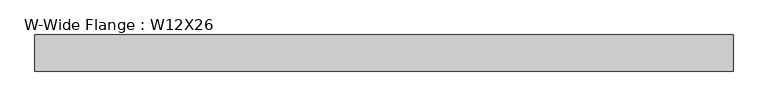
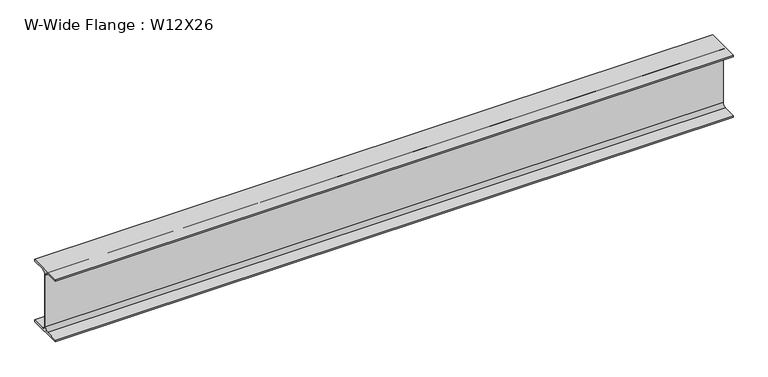
"""IFC4 building model written with IfcOpenShell, lengths in millimetres: beam geometry, W-Wide Flange : W12X26."""

import ifcopenshell
import ifcopenshell.guid

model = None  # the IFC model being written
_history = None  # IfcOwnerHistory: only IFC2X3 demands one
_inside = {}  # id of a spatial element -> (the spatial element, [elements in it])
_under = {}  # id of a project, library or spatial element -> (it, [spatial elements below it])
_declared = {}  # id of a project -> (the project, [libraries it declares])
_typed = {}  # id of a type object -> (the type object, [elements of that type])
_made_of = {}  # id of a material, layer set ... -> (it, [elements and type objects made of it])


def new_model(schema):
    """Start an empty IFC model of exactly this schema.

    Asked for "IFC4X3", IfcOpenShell would pick the latest addendum, in which some entities
    have other attributes; the version numbers below select the first issue.
    IFC2X3 requires an IfcOwnerHistory on every rooted entity: one is made here for all.
    """
    global model, _history
    if schema == "IFC4X3":
        model = ifcopenshell.file(schema_version=(4, 3, 0, 0))
    else:
        model = ifcopenshell.file(schema=schema)
    _inside.clear()
    _under.clear()
    _declared.clear()
    _typed.clear()
    _made_of.clear()
    _history = None
    if model.schema == "IFC2X3":
        org = make("IfcOrganization", Name="unknown")
        user = make(
            "IfcPersonAndOrganization",
            ThePerson=make("IfcPerson", FamilyName="unknown"),
            TheOrganization=org,
        )
        app = make(
            "IfcApplication",
            ApplicationDeveloper=org,
            Version="unknown",
            ApplicationFullName="unknown",
            ApplicationIdentifier="unknown",
        )
        _history = make(
            "IfcOwnerHistory",
            OwningUser=user,
            OwningApplication=app,
            ChangeAction="ADDED",
            CreationDate=0,
        )
    return model


def make(cls, **values):
    """One entity of the class cls with the attributes given. An attribute that is None is left unset."""
    return model.create_entity(
        cls, **{name: value for name, value in values.items() if value is not None}
    )


def rooted(cls, **values):
    """An entity with a GlobalId (a new one), such as an element, a storey or a relation."""
    return make(cls, GlobalId=ifcopenshell.guid.new(), OwnerHistory=_history, **values)


def si_unit(unit_type, name, prefix=None):
    """IfcSIUnit, for example si_unit("LENGTHUNIT", "METRE", prefix="MILLI")."""
    return make("IfcSIUnit", UnitType=unit_type, Prefix=prefix, Name=name)


def assignment(units):
    """IfcUnitAssignment: the units of a project."""
    return None if units is None else make("IfcUnitAssignment", Units=units)


def point(xyz):
    """IfcCartesianPoint."""
    return None if xyz is None else make("IfcCartesianPoint", Coordinates=xyz)


def direction(xyz):
    """IfcDirection."""
    return None if xyz is None else make("IfcDirection", DirectionRatios=xyz)


def frame(location, z_axis=None, x_axis=None):
    """IfcAxis2Placement3D, a coordinate frame: its origin and axes. An axis left out is left unset."""
    return make(
        "IfcAxis2Placement3D",
        Location=point(location),
        Axis=direction(z_axis),
        RefDirection=direction(x_axis),
    )


def frame_2d(location, x_axis=None):
    """IfcAxis2Placement2D, a coordinate frame in the plane: its origin and x axis."""
    return make(
        "IfcAxis2Placement2D", Location=point(location), RefDirection=direction(x_axis)
    )


def origin():
    """The frame at (0, 0, 0) with its axes left unset."""
    return frame((0.0, 0.0, 0.0))


def place(relative_to, where):
    """IfcLocalPlacement: puts the frame where relative to a parent placement (None: the world)."""
    return make(
        "IfcLocalPlacement", PlacementRelTo=relative_to, RelativePlacement=where
    )


def context(
    kind, dimensions, precision=None, world=None, true_north=None, identifier=None
):
    """IfcGeometricRepresentationContext, for example the 3D "Model" context."""
    return make(
        "IfcGeometricRepresentationContext",
        ContextIdentifier=identifier,
        ContextType=kind,
        CoordinateSpaceDimension=dimensions,
        Precision=precision,
        WorldCoordinateSystem=world,
        TrueNorth=true_north,
    )


def project(units=None, contexts=None):
    """IfcProject with its units and contexts."""
    return rooted(
        "IfcProject",
        Name="project",
        RepresentationContexts=contexts,
        UnitsInContext=assignment(units),
    )


def spatial(cls, under=None, at=None, **own):
    """A site, building, storey or space (cls), placed at a placement, below another one or the project."""
    s = rooted(cls, ObjectPlacement=at, **own)
    if under is not None:
        _under.setdefault(under.id(), (under, []))[1].append(s)
    return s


def polyline(points):
    """IfcPolyline through the points."""
    return make("IfcPolyline", Points=[point(p) for p in points])


def circle_curve(where, radius):
    """IfcCircle in the frame where."""
    return make("IfcCircle", Position=where, Radius=radius)


def trimmed(basis, trim1, trim2, sense, master):
    """IfcTrimmedCurve: the piece of a basis curve between two trims."""
    return make(
        "IfcTrimmedCurve",
        BasisCurve=basis,
        Trim1=trim1,
        Trim2=trim2,
        SenseAgreement=sense,
        MasterRepresentation=master,
    )


def segment(curve, same_sense, transition):
    """IfcCompositeCurveSegment."""
    return make(
        "IfcCompositeCurveSegment",
        Transition=transition,
        SameSense=same_sense,
        ParentCurve=curve,
    )


def composite_curve(segments, self_intersect=None):
    """IfcCompositeCurve: segments joined end to end."""
    return make("IfcCompositeCurve", Segments=segments, SelfIntersect=self_intersect)


def outline(outer, holes=None, kind="AREA"):
    """IfcArbitraryClosedProfileDef: a profile drawn as a closed curve; with holes, ...WithVoids."""
    if holes is None:
        return make("IfcArbitraryClosedProfileDef", ProfileType=kind, OuterCurve=outer)
    return make(
        "IfcArbitraryProfileDefWithVoids",
        ProfileType=kind,
        OuterCurve=outer,
        InnerCurves=holes,
    )


def extrude(swept, where, along, depth):
    """IfcExtrudedAreaSolid: the profile swept, set in the frame where, extruded along a direction by depth."""
    return make(
        "IfcExtrudedAreaSolid",
        SweptArea=swept,
        Position=where,
        ExtrudedDirection=direction(along),
        Depth=depth,
    )


def shape(context_of_items, identifier, shape_type, items):
    """IfcShapeRepresentation: the items that make up one representation, for example the "Body"."""
    return make(
        "IfcShapeRepresentation",
        ContextOfItems=context_of_items,
        RepresentationIdentifier=identifier,
        RepresentationType=shape_type,
        Items=items,
    )


def source(mapping_origin, context_of_items, identifier, shape_type, items):
    """IfcRepresentationMap: a shape defined once, which mapped items show again and again."""
    return make(
        "IfcRepresentationMap",
        MappingOrigin=mapping_origin,
        MappedRepresentation=shape(context_of_items, identifier, shape_type, items),
    )


def transform(
    local_origin,
    x_axis=None,
    y_axis=None,
    z_axis=None,
    scale=None,
    scale2=None,
    scale3=None,
    uniform=True,
):
    """IfcCartesianTransformationOperator3D, or its non-uniform kind. x_axis, y_axis, z_axis: its Axis1, 2, 3."""
    if uniform:
        return make(
            "IfcCartesianTransformationOperator3D",
            Axis1=direction(x_axis),
            Axis2=direction(y_axis),
            LocalOrigin=point(local_origin),
            Scale=scale,
            Axis3=direction(z_axis),
        )
    return make(
        "IfcCartesianTransformationOperator3DnonUniform",
        Axis1=direction(x_axis),
        Axis2=direction(y_axis),
        LocalOrigin=point(local_origin),
        Scale=scale,
        Axis3=direction(z_axis),
        Scale2=scale2,
        Scale3=scale3,
    )


def mapped(mapping_source, mapping_target):
    """IfcMappedItem: shows the shape of a source again, moved by a transform."""
    return make(
        "IfcMappedItem", MappingSource=mapping_source, MappingTarget=mapping_target
    )


def made_of(thing, what):
    """Note that an element or type object is made of a material, layer set ...; save() writes the relation."""
    if what is not None:
        _made_of.setdefault(what.id(), (what, []))[1].append(thing)
    return thing


def element(
    cls,
    number,
    at=None,
    inside=None,
    cuts=None,
    type_object=None,
    material=None,
    context=None,
    identifier="Body",
    shape_type=None,
    held_by="IfcProductDefinitionShape",
    body=None,
    shapes=None,
    **own,
):
    """One element of the class cls, such as IfcWall. Its Tag is "e" and its number.

    at: its placement. inside: the storey or other place that contains it. cuts: it is an
    opening in that element (IfcRelVoidsElement). A single representation is given by context,
    identifier, shape_type and body (its items); several are given by shapes. held_by: the class
    of the entity that holds the representations. save() writes the other relations.
    """
    e = rooted(cls, Tag="e%d" % number, ObjectPlacement=at, **own)
    if body is not None:
        shapes = [shape(context, identifier, shape_type, body)]
    if shapes is not None:
        e.Representation = make(held_by, Representations=shapes)
    if inside is not None:
        _inside.setdefault(inside.id(), (inside, []))[1].append(e)
    if cuts is not None:
        rooted(
            "IfcRelVoidsElement", RelatingBuildingElement=cuts, RelatedOpeningElement=e
        )
    if type_object is not None:
        _typed.setdefault(type_object.id(), (type_object, []))[1].append(e)
    return made_of(e, material)


def aggregate(whole, parts):
    """IfcRelAggregates: a whole, such as a stair, and the parts it consists of."""
    return rooted("IfcRelAggregates", RelatingObject=whole, RelatedObjects=parts)


def save(model, path):
    """Write the relations noted so far, then the file.

    IfcRelAggregates (storeys below a building ...), IfcRelContainedInSpatialStructure (elements
    in a storey), IfcRelDefinesByType, IfcRelAssociatesMaterial and IfcRelDeclares: one each for
    every whole, place, type object, material and project.
    """
    for whole, parts in _under.values():
        aggregate(whole, parts)
    for where, things in _inside.values():
        rooted(
            "IfcRelContainedInSpatialStructure",
            RelatedElements=things,
            RelatingStructure=where,
        )
    for kind, things in _typed.values():
        rooted("IfcRelDefinesByType", RelatedObjects=things, RelatingType=kind)
    for what, things in _made_of.values():
        rooted("IfcRelAssociatesMaterial", RelatedObjects=things, RelatingMaterial=what)
    for by, libraries in _declared.values():
        rooted("IfcRelDeclares", RelatingContext=by, RelatedDefinitions=libraries)
    model.write(path)


def w_wide_flange_w12x26_4149ab62(model_context):
    return source(origin(), model_context, "Body", "SweptSolid", [
        extrude(outline(composite_curve([segment(polyline([(82.4011719, -145.5539063), (82.4011719, -155.178125), (-82.4011719, -155.178125), (-82.4011719, -145.5539063), (-20.2902344, -145.5539063)]), True, "CONTINUOUS"), segment(trimmed(circle_curve(frame_2d((-20.2902344, -128.190625)), 17.3632812), [point((-20.2902344, -145.5539063))], [point((-2.9269531, -128.190625))], True, "CARTESIAN"), True, "CONTINUOUS"), segment(polyline([(-2.9269531, -128.190625), (-2.9269531, 128.190625)]), True, "CONTINUOUS"), segment(trimmed(circle_curve(frame_2d((-20.2902344, 128.190625)), 17.3632812), [point((-2.9269531, 128.190625))], [point((-20.2902344, 145.5539062))], True, "CARTESIAN"), True, "CONTINUOUS"), segment(polyline([(-20.2902344, 145.5539062), (-82.4011719, 145.5539062), (-82.4011719, 155.178125), (82.4011719, 155.178125), (82.4011719, 145.5539062), (20.2902344, 145.5539062)]), True, "CONTINUOUS"), segment(trimmed(circle_curve(frame_2d((20.2902344, 128.190625)), 17.3632812), [point((20.2902344, 145.5539062))], [point((2.9269531, 128.190625))], True, "CARTESIAN"), True, "CONTINUOUS"), segment(polyline([(2.9269531, 128.190625), (2.9269531, -128.190625)]), True, "CONTINUOUS"), segment(trimmed(circle_curve(frame_2d((20.2902344, -128.190625)), 17.3632812), [point((2.9269531, -128.190625))], [point((20.2902344, -145.5539063))], True, "CARTESIAN"), True, "CONTINUOUS"), segment(polyline([(20.2902344, -145.5539063), (82.4011719, -145.5539063)]), True, "CONTINUOUS")], self_intersect=False)), frame((-1535.865688, 0.0, 0.0), z_axis=(1.0, 0.0, 0.0), x_axis=(0.0, 1.0, 0.0)), (0.0, 0.0, 1.0), 3186.0313761),
    ])


if __name__ == "__main__":
    model = new_model("IFC4")
    model_context = context("Model", 3, world=origin())
    ifc_project = project(units=[si_unit("LENGTHUNIT", "METRE", prefix="MILLI")], contexts=[model_context])
    site = spatial("IfcSite", under=ifc_project)
    building = spatial("IfcBuilding", under=site)
    placement = place(None, origin())
    w_wide_flange_w12x26_shape = w_wide_flange_w12x26_4149ab62(model_context)
    element("IfcBeam", 1, ObjectType="W-Wide Flange : W12X26", at=placement, inside=building, context=model_context, shape_type="MappedRepresentation", body=[
        mapped(w_wide_flange_w12x26_shape, transform((0.0, 0.0, 0.0), x_axis=(1.0, 0.0, 0.0), y_axis=(0.0, 1.0, 0.0), z_axis=(0.0, 0.0, 1.0))),
    ])
    save(model, "model.ifc")

# Revit data of these elements
# Type "W-Wide Flange : W12X26"
#   Assembly Code = "B10"
#   W = 26
#   Length [instance default] = 5' - 0"
#   bf = 0' - 6 125/256"
#   d = 1' - 0 7/32"
#   k = 0' - 1 1/16"
#   k2 = 0' - 0 175/256"
#   tf = 0' - 0 97/256"
#   tw = 0' - 0 59/256"
#   A = 0.053125 SF
#   Structural Material [instance default] = none
# Element 1 (IfcBeam, "W-Wide Flange : W12X26")
#   Structural Material = Dark metal
#   Materials on its faces: "Dark metal"
# Materials
#   "Dark metal": class "Generic", colour RGB 44 29 29, transparency 0, Cost = 0
